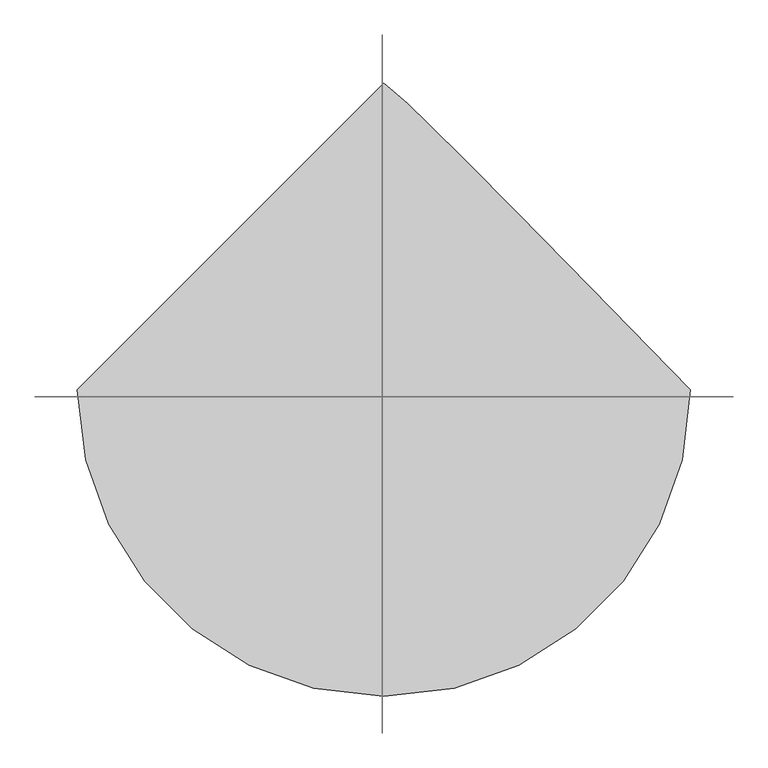
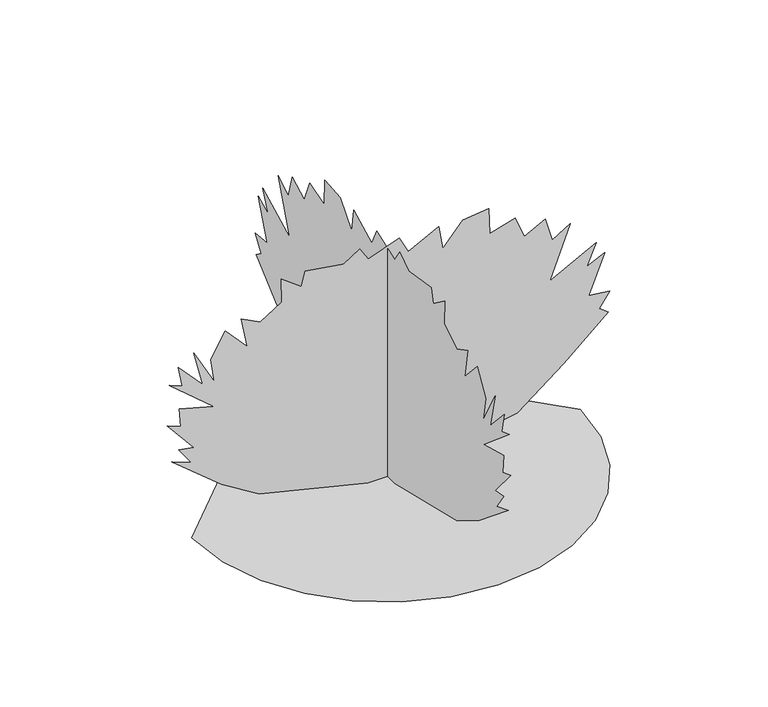
"""IFC4 building model written with IfcOpenShell, lengths in millimetres: proxy geometry, yew 26768 : yew 26768."""

import ifcopenshell
import ifcopenshell.guid

model = None  # the IFC model being written
_history = None  # IfcOwnerHistory: only IFC2X3 demands one
_inside = {}  # id of a spatial element -> (the spatial element, [elements in it])
_under = {}  # id of a project, library or spatial element -> (it, [spatial elements below it])
_declared = {}  # id of a project -> (the project, [libraries it declares])
_typed = {}  # id of a type object -> (the type object, [elements of that type])
_made_of = {}  # id of a material, layer set ... -> (it, [elements and type objects made of it])


def new_model(schema):
    """Start an empty IFC model of exactly this schema.

    Asked for "IFC4X3", IfcOpenShell would pick the latest addendum, in which some entities
    have other attributes; the version numbers below select the first issue.
    IFC2X3 requires an IfcOwnerHistory on every rooted entity: one is made here for all.
    """
    global model, _history
    if schema == "IFC4X3":
        model = ifcopenshell.file(schema_version=(4, 3, 0, 0))
    else:
        model = ifcopenshell.file(schema=schema)
    _inside.clear()
    _under.clear()
    _declared.clear()
    _typed.clear()
    _made_of.clear()
    _history = None
    if model.schema == "IFC2X3":
        org = make("IfcOrganization", Name="unknown")
        user = make(
            "IfcPersonAndOrganization",
            ThePerson=make("IfcPerson", FamilyName="unknown"),
            TheOrganization=org,
        )
        app = make(
            "IfcApplication",
            ApplicationDeveloper=org,
            Version="unknown",
            ApplicationFullName="unknown",
            ApplicationIdentifier="unknown",
        )
        _history = make(
            "IfcOwnerHistory",
            OwningUser=user,
            OwningApplication=app,
            ChangeAction="ADDED",
            CreationDate=0,
        )
    return model


def make(cls, **values):
    """One entity of the class cls with the attributes given. An attribute that is None is left unset."""
    return model.create_entity(
        cls, **{name: value for name, value in values.items() if value is not None}
    )


def rooted(cls, **values):
    """An entity with a GlobalId (a new one), such as an element, a storey or a relation."""
    return make(cls, GlobalId=ifcopenshell.guid.new(), OwnerHistory=_history, **values)


def si_unit(unit_type, name, prefix=None):
    """IfcSIUnit, for example si_unit("LENGTHUNIT", "METRE", prefix="MILLI")."""
    return make("IfcSIUnit", UnitType=unit_type, Prefix=prefix, Name=name)


def assignment(units):
    """IfcUnitAssignment: the units of a project."""
    return None if units is None else make("IfcUnitAssignment", Units=units)


def point(xyz):
    """IfcCartesianPoint."""
    return None if xyz is None else make("IfcCartesianPoint", Coordinates=xyz)


def direction(xyz):
    """IfcDirection."""
    return None if xyz is None else make("IfcDirection", DirectionRatios=xyz)


def frame(location, z_axis=None, x_axis=None):
    """IfcAxis2Placement3D, a coordinate frame: its origin and axes. An axis left out is left unset."""
    return make(
        "IfcAxis2Placement3D",
        Location=point(location),
        Axis=direction(z_axis),
        RefDirection=direction(x_axis),
    )


def origin():
    """The frame at (0, 0, 0) with its axes left unset."""
    return frame((0.0, 0.0, 0.0))


def place(relative_to, where):
    """IfcLocalPlacement: puts the frame where relative to a parent placement (None: the world)."""
    return make(
        "IfcLocalPlacement", PlacementRelTo=relative_to, RelativePlacement=where
    )


def context(
    kind, dimensions, precision=None, world=None, true_north=None, identifier=None
):
    """IfcGeometricRepresentationContext, for example the 3D "Model" context."""
    return make(
        "IfcGeometricRepresentationContext",
        ContextIdentifier=identifier,
        ContextType=kind,
        CoordinateSpaceDimension=dimensions,
        Precision=precision,
        WorldCoordinateSystem=world,
        TrueNorth=true_north,
    )


def project(units=None, contexts=None):
    """IfcProject with its units and contexts."""
    return rooted(
        "IfcProject",
        Name="project",
        RepresentationContexts=contexts,
        UnitsInContext=assignment(units),
    )


def spatial(cls, under=None, at=None, **own):
    """A site, building, storey or space (cls), placed at a placement, below another one or the project."""
    s = rooted(cls, ObjectPlacement=at, **own)
    if under is not None:
        _under.setdefault(under.id(), (under, []))[1].append(s)
    return s


def point_list(points):
    """IfcCartesianPointList2D or 3D."""
    cls = (
        "IfcCartesianPointList2D" if len(points[0]) == 2 else "IfcCartesianPointList3D"
    )
    return make(cls, CoordList=points)


def triangles(points, corners, closed=None, point_numbers=None):
    """IfcTriangulatedFaceSet: each triangle names its three corners, points numbered from 1."""
    return make(
        "IfcTriangulatedFaceSet",
        Coordinates=point_list(points),
        Closed=closed,
        CoordIndex=corners,
        PnIndex=point_numbers,
    )


def shape(context_of_items, identifier, shape_type, items):
    """IfcShapeRepresentation: the items that make up one representation, for example the "Body"."""
    return make(
        "IfcShapeRepresentation",
        ContextOfItems=context_of_items,
        RepresentationIdentifier=identifier,
        RepresentationType=shape_type,
        Items=items,
    )


def source(mapping_origin, context_of_items, identifier, shape_type, items):
    """IfcRepresentationMap: a shape defined once, which mapped items show again and again."""
    return make(
        "IfcRepresentationMap",
        MappingOrigin=mapping_origin,
        MappedRepresentation=shape(context_of_items, identifier, shape_type, items),
    )


def transform(
    local_origin,
    x_axis=None,
    y_axis=None,
    z_axis=None,
    scale=None,
    scale2=None,
    scale3=None,
    uniform=True,
):
    """IfcCartesianTransformationOperator3D, or its non-uniform kind. x_axis, y_axis, z_axis: its Axis1, 2, 3."""
    if uniform:
        return make(
            "IfcCartesianTransformationOperator3D",
            Axis1=direction(x_axis),
            Axis2=direction(y_axis),
            LocalOrigin=point(local_origin),
            Scale=scale,
            Axis3=direction(z_axis),
        )
    return make(
        "IfcCartesianTransformationOperator3DnonUniform",
        Axis1=direction(x_axis),
        Axis2=direction(y_axis),
        LocalOrigin=point(local_origin),
        Scale=scale,
        Axis3=direction(z_axis),
        Scale2=scale2,
        Scale3=scale3,
    )


def mapped(mapping_source, mapping_target):
    """IfcMappedItem: shows the shape of a source again, moved by a transform."""
    return make(
        "IfcMappedItem", MappingSource=mapping_source, MappingTarget=mapping_target
    )


def made_of(thing, what):
    """Note that an element or type object is made of a material, layer set ...; save() writes the relation."""
    if what is not None:
        _made_of.setdefault(what.id(), (what, []))[1].append(thing)
    return thing


def element(
    cls,
    number,
    at=None,
    inside=None,
    cuts=None,
    type_object=None,
    material=None,
    context=None,
    identifier="Body",
    shape_type=None,
    held_by="IfcProductDefinitionShape",
    body=None,
    shapes=None,
    **own,
):
    """One element of the class cls, such as IfcWall. Its Tag is "e" and its number.

    at: its placement. inside: the storey or other place that contains it. cuts: it is an
    opening in that element (IfcRelVoidsElement). A single representation is given by context,
    identifier, shape_type and body (its items); several are given by shapes. held_by: the class
    of the entity that holds the representations. save() writes the other relations.
    """
    e = rooted(cls, Tag="e%d" % number, ObjectPlacement=at, **own)
    if body is not None:
        shapes = [shape(context, identifier, shape_type, body)]
    if shapes is not None:
        e.Representation = make(held_by, Representations=shapes)
    if inside is not None:
        _inside.setdefault(inside.id(), (inside, []))[1].append(e)
    if cuts is not None:
        rooted(
            "IfcRelVoidsElement", RelatingBuildingElement=cuts, RelatedOpeningElement=e
        )
    if type_object is not None:
        _typed.setdefault(type_object.id(), (type_object, []))[1].append(e)
    return made_of(e, material)


def aggregate(whole, parts):
    """IfcRelAggregates: a whole, such as a stair, and the parts it consists of."""
    return rooted("IfcRelAggregates", RelatingObject=whole, RelatedObjects=parts)


def save(model, path):
    """Write the relations noted so far, then the file.

    IfcRelAggregates (storeys below a building ...), IfcRelContainedInSpatialStructure (elements
    in a storey), IfcRelDefinesByType, IfcRelAssociatesMaterial and IfcRelDeclares: one each for
    every whole, place, type object, material and project.
    """
    for whole, parts in _under.values():
        aggregate(whole, parts)
    for where, things in _inside.values():
        rooted(
            "IfcRelContainedInSpatialStructure",
            RelatedElements=things,
            RelatingStructure=where,
        )
    for kind, things in _typed.values():
        rooted("IfcRelDefinesByType", RelatedObjects=things, RelatingType=kind)
    for what, things in _made_of.values():
        rooted("IfcRelAssociatesMaterial", RelatedObjects=things, RelatingMaterial=what)
    for by, libraries in _declared.values():
        rooted("IfcRelDeclares", RelatingContext=by, RelatedDefinitions=libraries)
    model.write(path)


def entourage_1708232a(model_context):
    return source(origin(), model_context, "Body", "Tessellation", [
        triangles([(-552.1733454, 0.0, 5.4e-06), (-537.5734008, -126.5215106, 5.4e-06), (-496.001229, -242.7110573, 5.4e-06), (-430.7790836, -345.2394648, 5.4e-06), (-345.2394648, -430.7790836, 5.4e-06), (-242.7110573, -496.001229, 5.4e-06), (-126.5212562, -537.5734008, 5.4e-06), (2.41e-05, -552.1733454, 5.4e-06), (126.5215106, -537.5734008, 5.4e-06), (242.7110573, -496.001229, 5.4e-06), (345.2394648, -430.7790836, 5.4e-06), (430.7790836, -345.2394648, 5.4e-06), (496.001229, -242.7110573, 5.4e-06), (537.5734008, -126.5212562, 5.4e-06), (552.1733454, 4.83e-05, 5.4e-06), (372.7273582, 184.0654909, 5.4e-06), (239.6978509, 319.5854711, 5.4e-06), (145.3449528, 414.6475465, 5.4e-06), (81.9343338, 477.3474621, 5.4e-06), (41.7301836, 515.775131, 5.4e-06), (16.9973058, 538.0179231, 5.4e-06), (-7.24e-05, 552.1733454, 5.4e-06), (-57.9623142, -12.396627, 5.21e-05), (-367.0047423, -12.396652, 75.5734076), (-474.5509031, -12.396652, 142.0056127), (-616.6665018, -12.396652, 259.1080397), (-561.3351408, -12.396652, 237.5164979), (-596.4227157, -12.396652, 287.4493694), (-553.2375973, -12.396652, 279.351844), (-628.8127808, -12.396652, 371.1195348), (-591.025189, -12.396652, 356.2757824), (-595.0739608, -12.396652, 410.2558814), (-496.5574814, -12.396652, 383.2658137), (-623.412747, -12.3966781, 491.2285552), (-585.6276987, -12.3966781, 476.3822594), (-597.7714342, -12.3966781, 535.7623921), (-527.5962845, -12.3966781, 460.1872087), (-553.2375973, -12.3966781, 564.1011784), (-495.2087265, -12.3966781, 457.4897352), (-506.0037435, -12.3966781, 527.6648849), (-464.1699234, -12.3966781, 599.1887532), (-402.0923172, -12.3966781, 530.3649018), (-418.2848245, -12.3966781, 619.4325394), (-364.3047255, -12.3966781, 591.091246), (-303.5758378, -12.3966781, 630.2275927), (-304.9245564, -12.3966781, 699.0539875), (-248.2454578, -12.3966781, 657.2201311), (-237.4491873, -12.3966781, 699.0539875), (-126.787955, -12.3966781, 681.5102182), (-82.2536094, -12.3966781, 711.2002665), (-57.9623142, -12.3966781, 673.4126747), (29.7568728, -12.3966781, 705.8027761), (55.3245209, -12.3966781, 655.0738958), (143.2032231, -12.3966781, 700.044552), (153.8874819, -12.3966781, 630.387612), (210.5935046, -12.3966781, 696.3564777), (284.8179166, -12.3966781, 704.4514778), (287.5154082, -12.3966781, 628.8788378), (360.3905748, -12.3966781, 649.1226603), (386.0318876, -12.3966781, 584.3450008), (445.4120204, -12.3966781, 616.7325588), (465.6532994, -12.3966781, 546.5574091), (515.5871701, -12.3966781, 578.9474742), (457.5557559, -12.396652, 426.4509321), (589.8110916, -12.3966781, 495.2747835), (562.8184805, -12.396652, 433.197141), (614.1011061, -12.3966781, 457.4897352), (568.2185143, -12.396652, 344.1295034), (628.9474382, -12.396652, 336.0319599), (597.9085988, -12.396652, 294.1956146), (623.5474045, -12.396652, 275.3030723), (498.0433645, -12.396652, 164.6420943), (365.7880651, -12.396652, 62.0781285), (289.9233281, -12.396652, 47.6486405), (164.5613216, -12.396652, 15.2766327), (36.5046395, -12.396627, 1.4e-05), (-3.3569921, -47.7068037, 4.09e-05), (-3.3569921, -356.74821, 75.5734076), (-3.3569921, -464.2969142, 142.0056127), (-3.3569921, -606.4099694, 259.1080397), (-3.3569921, -551.0786084, 237.5164979), (-3.3569921, -586.1687267, 287.4493694), (-3.3569921, -542.9836083, 279.351844), (-3.3569921, -618.5562847, 371.1195348), (-3.3569921, -580.7686566, 356.2757824), (-3.3569921, -584.8174284, 410.2558814), (-3.3569921, -486.3034925, 383.2658137), (-3.3569921, -613.1587944, 491.2285552), (-3.3569921, -575.3711663, 476.3822594), (-3.3569669, -587.5174453, 535.7623921), (-3.3569921, -517.3422956, 460.1872087), (-3.3569669, -542.9836083, 564.1011784), (-3.3569921, -484.9522305, 457.4897352), (-3.3569921, -495.7497545, 527.6648849), (-3.3569669, -453.913391, 599.1887532), (-3.3569921, -391.8357848, 530.3649018), (-3.3569669, -408.0308355, 619.4325394), (-3.3569921, -354.0481931, 591.091246), (-3.3569921, -293.3193054, 630.2275927), (-3.3569669, -294.6705856, 699.0539875), (-3.3569921, -237.9897067, 657.2201311), (-3.3569669, -227.1936905, 699.0539875), (-3.3569921, -116.5324491, 681.5102182), (-3.3569921, -71.9981035, 711.2002665), (-3.3569921, -47.7068037, 673.4126747), (-3.3569921, 40.0126331, 705.8027761), (-3.3569921, 65.5800314, 655.0738958), (-3.3569921, 153.458729, 700.044552), (-3.3569921, 164.1429969, 630.387612), (-3.3569921, 220.8490196, 696.3564777), (-3.3569921, 295.0719056, 704.4514778), (-3.3569921, 297.7719224, 628.8788378), (-3.3569921, 370.6471072, 649.1226603), (-3.3569921, 396.28842, 584.3450008), (-3.3569921, 455.6660093, 616.7325588), (-3.3569921, 475.9098318, 546.5574091), (-3.3569921, 525.8411591, 578.9474742), (-3.3569921, 467.8122883, 426.4509321), (-3.3569921, 600.0650442, 495.2747835), (-3.3569921, 573.0750129, 433.197141), (-3.3569921, 624.3576021, 457.4897352), (-3.3569921, 578.4725032, 344.1295034), (-3.3569921, 639.2013908, 336.0319599), (-3.3569921, 608.1625877, 294.1956146), (-3.3569921, 633.8039005, 275.3030723), (-3.3570177, 508.2973535, 164.6420943), (-3.3570177, 376.0445975, 62.0781285), (-3.3570177, 300.1798423, 47.6486405), (-3.3569921, 174.8168366, 15.2766327), (-3.3569921, 46.7601454, 0.0)], [[21, 22, 1], [20, 21, 1], [19, 20, 1], [18, 19, 1], [17, 18, 1], [17, 1, 2], [17, 2, 3], [17, 3, 4], [16, 17, 4], [16, 4, 5], [16, 5, 6], [16, 6, 7], [16, 7, 8], [16, 8, 9], [16, 9, 10], [16, 10, 11], [16, 11, 12], [15, 16, 12], [14, 15, 12], [13, 14, 12], [37, 38, 39], [25, 26, 27], [33, 34, 35], [29, 30, 31], [35, 36, 37], [33, 35, 37], [62, 63, 64], [64, 65, 66], [66, 67, 68], [27, 28, 29], [42, 43, 44], [45, 46, 47], [68, 69, 70], [33, 37, 39], [31, 32, 33], [53, 54, 55], [40, 41, 42], [60, 61, 62], [70, 71, 72], [29, 31, 33], [39, 40, 42], [56, 57, 58], [49, 50, 51], [55, 56, 58], [64, 66, 68], [47, 48, 49], [58, 59, 60], [51, 52, 53], [60, 62, 64], [68, 70, 72], [64, 68, 72], [64, 72, 73], [64, 73, 74], [25, 27, 29], [25, 29, 33], [24, 25, 33], [23, 24, 33], [64, 74, 75], [60, 64, 75], [58, 60, 75], [55, 58, 75], [55, 75, 76], [53, 55, 76], [53, 76, 23], [53, 23, 33], [51, 53, 33], [49, 51, 33], [47, 49, 33], [45, 47, 33], [33, 39, 42], [45, 33, 42], [44, 45, 42], [91, 92, 93], [79, 80, 81], [87, 88, 89], [83, 84, 85], [89, 90, 91], [87, 89, 91], [116, 117, 118], [118, 119, 120], [120, 121, 122], [81, 82, 83], [96, 97, 98], [99, 100, 101], [122, 123, 124], [87, 91, 93], [85, 86, 87], [107, 108, 109], [94, 95, 96], [114, 115, 116], [124, 125, 126], [83, 85, 87], [93, 94, 96], [110, 111, 112], [103, 104, 105], [109, 110, 112], [118, 120, 122], [101, 102, 103], [112, 113, 114], [105, 106, 107], [114, 116, 118], [122, 124, 126], [118, 122, 126], [118, 126, 127], [118, 127, 128], [79, 81, 83], [79, 83, 87], [78, 79, 87], [77, 78, 87], [118, 128, 129], [114, 118, 129], [112, 114, 129], [109, 112, 129], [109, 129, 130], [107, 109, 130], [107, 130, 77], [107, 77, 87], [105, 107, 87], [103, 105, 87], [101, 103, 87], [99, 101, 87], [87, 93, 96], [99, 87, 96], [98, 99, 96]], closed=False),
    ])


if __name__ == "__main__":
    model = new_model("IFC4")
    model_context = context("Model", 3, world=origin())
    ifc_project = project(units=[si_unit("LENGTHUNIT", "METRE", prefix="MILLI")], contexts=[model_context])
    site = spatial("IfcSite", under=ifc_project)
    building = spatial("IfcBuilding", under=site)
    placement = place(None, origin())
    entourage_shape = entourage_1708232a(model_context)
    element("IfcBuildingElementProxy", 1, Name="yew 26768 : yew 26768", ObjectType="yew 26768 : yew 26768", at=placement, inside=building, context=model_context, shape_type="MappedRepresentation", body=[
        mapped(entourage_shape, transform((0.0, 0.0, 0.0), x_axis=(1.0, 0.0, 0.0), y_axis=(0.0, 1.0, 0.0), z_axis=(0.0, 0.0, 1.0))),
    ])
    save(model, "model.ifc")

# Revit data of these elements
# Type "yew 26768 : yew 26768"
#   built-in parameter 1005195 = "RPC-16-FWJ8-ELQ0-EHM0-2000-ST1L-LVER-AU"
#   Height = 0
